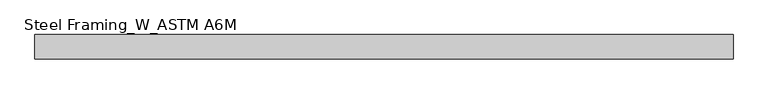
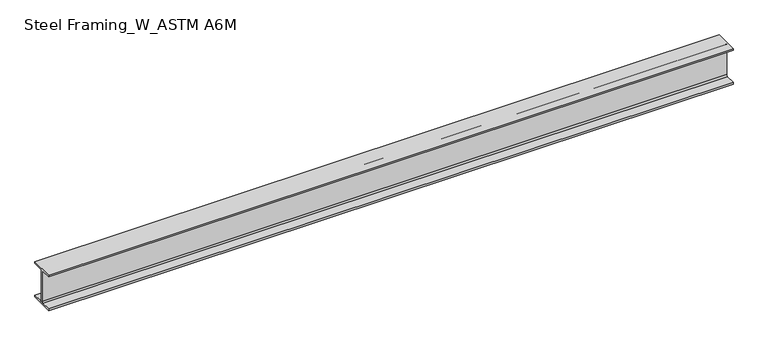
"""IFC4 building model written with IfcOpenShell, lengths in millimetres: beam geometry, Steel Framing_W_ASTM A6M : H_SB_AR_S02_W200x31.3_B6."""

from ifc_helpers import new_model, si_unit, point, frame, frame_2d, origin, place, context, project, spatial, polyline, circle_curve, trimmed, segment, composite_curve, outline, extrude, source, transform, mapped, element, save


def steel_framing_w_astm_a6m_fd2852ff(model_context):
    return source(origin(), model_context, "Body", "SweptSolid", [
        extrude(outline(composite_curve([segment(polyline([(67.0, -94.8), (67.0, -105.0), (-67.0, -105.0), (-67.0, -94.8), (-10.775, -94.8)]), True, "CONTINUOUS"), segment(trimmed(circle_curve(frame_2d((-10.775, -87.2)), 7.6), [point((-10.775, -94.8))], [point((-3.175, -87.2))], True, "CARTESIAN"), True, "CONTINUOUS"), segment(polyline([(-3.175, -87.2), (-3.175, 87.2)]), True, "CONTINUOUS"), segment(trimmed(circle_curve(frame_2d((-10.775, 87.2)), 7.6), [point((-3.175, 87.2))], [point((-10.775, 94.8))], True, "CARTESIAN"), True, "CONTINUOUS"), segment(polyline([(-10.775, 94.8), (-67.0, 94.8), (-67.0, 105.0), (67.0, 105.0), (67.0, 94.8), (10.775, 94.8)]), True, "CONTINUOUS"), segment(trimmed(circle_curve(frame_2d((10.775, 87.2)), 7.6), [point((10.775, 94.8))], [point((3.175, 87.2))], True, "CARTESIAN"), True, "CONTINUOUS"), segment(polyline([(3.175, 87.2), (3.175, -87.2)]), True, "CONTINUOUS"), segment(trimmed(circle_curve(frame_2d((10.775, -87.2)), 7.6), [point((3.175, -87.2))], [point((10.775, -94.8))], True, "CARTESIAN"), True, "CONTINUOUS"), segment(polyline([(10.775, -94.8), (67.0, -94.8)]), True, "CONTINUOUS")], self_intersect=False)), frame((-1920.3, 0.0, 0.0), z_axis=(1.0, 0.0, 0.0), x_axis=(0.0, 1.0, 0.0)), (0.0, 0.0, 1.0), 3840.6),
    ])


if __name__ == "__main__":
    model = new_model("IFC4")
    model_context = context("Model", 3, world=origin())
    ifc_project = project(units=[si_unit("LENGTHUNIT", "METRE", prefix="MILLI")], contexts=[model_context])
    site = spatial("IfcSite", under=ifc_project)
    building = spatial("IfcBuilding", under=site)
    placement = place(None, origin())
    steel_framing_w_astm_a6m_shape = steel_framing_w_astm_a6m_fd2852ff(model_context)
    element("IfcBeam", 1, ObjectType="Steel Framing_W_ASTM A6M : H_SB_AR_S02_W200x31.3_B6", at=placement, inside=building, context=model_context, shape_type="MappedRepresentation", body=[
        mapped(steel_framing_w_astm_a6m_shape, transform((0.0, 0.0, 0.0), x_axis=(1.0, 0.0, 0.0), y_axis=(0.0, 1.0, 0.0), z_axis=(0.0, 0.0, 1.0))),
    ])
    save(model, "model.ifc")

# Revit data of these elements
# Type "Steel Framing_W_ASTM A6M : H_SB_AR_S02_W200x31.3_B6"
#   Type Mark = "B6"
#   Section Name Key = "W8x21"
#   Width = 13.4 cm
#   Web Thickness = 0.635 cm
#   Web Fillet = 0.76 cm
#   Warping Constant = 40800.0 cm⁶
#   Torsional Moment of Inertia = 11.70 cm⁴
#   Section Area = 39.7 cm²
#   Plastic Modulus weak axis = 93.2 cm³
#   Plastic Modulus strong axis = 334.0 cm³
#   Perimeter = 0.93 m²/m
#   Nominal Weight = 31.30 kgf/m
#   Moment of Inertia weak axis = 407.00 cm⁴
#   Moment of Inertia strong axis = 3130.00 cm⁴
#   Height = 21.0 cm
#   Flange Thickness = 1.02 cm
#   Elastic Modulus weak axis = 60.8 cm³
#   Elastic Modulus strong axis = 298.0 cm³
#   Centroid Vertical = 10.5 cm
#   Centroid Horizontal = 6.7 cm
#   Length [instance default] = 1500 mm
#   Structural Material [instance default] = Steel, 45-345
#   Bolt Spacing = 0
#   Assembly Code = ""
# Element 1 (IfcBeam, "Steel Framing_W_ASTM A6M : H_SB_AR_S02_W200x31.3_B6")
#   Materials on its faces: "Steel, 45-345"
# Materials
#   "Steel, 45-345": class "Metal", colour RGB 189 187 185, transparency 0, Description = "Steel 345 MPa", Cost = 0
